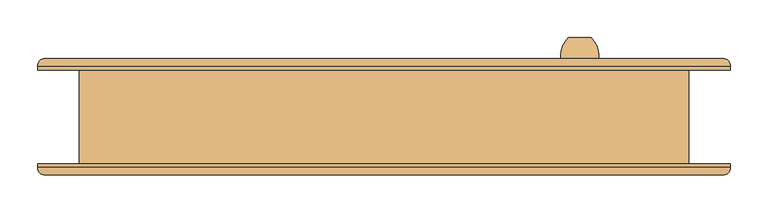
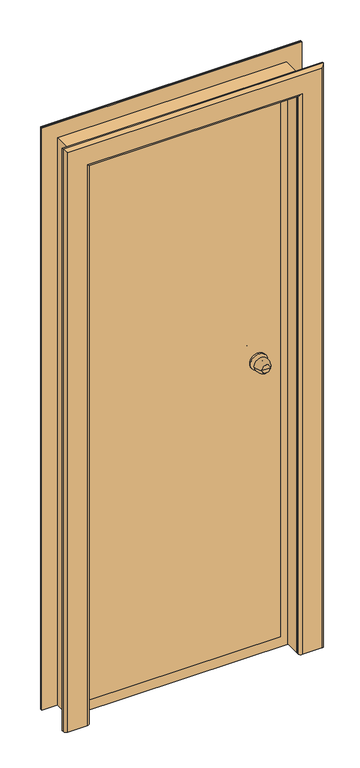
"""IFC4 building model written with IfcOpenShell, lengths in millimetres: door geometry, Наружная дверь 1-Навесная - Один проем наружу с порогом - 31173-2003 : ДСН КЛН  М1 УЗ 2100-810 ГОСТ 31173-2003."""

from ifc_helpers import new_model, si_unit, point, frame, origin, place, context, project, spatial, polyline, circle_curve, ellipse_curve, trimmed, outline, extrude, faceted_brep, source, transform, mapped, element, save
from ifc_brep_helpers import plane_surface, cylinder_surface, revolved_surface, advanced_brep


def door_b60437f9(model_context):
    return source(origin(), model_context, "Body", "SolidModel", [
        advanced_brep(
        [(245.0, 105.5, 1100.0), (275.0, 105.5, 1100.0), (260.0, 105.5, 1100.0), (235.0, 75.5, 1100.0), (285.0, 75.5, 1100.0), (242.0, 75.5, 1100.0), (278.0, 75.5, 1100.0), (250.0, 67.5, 1100.0), (270.0, 67.5, 1100.0), (250.0, 61.5, 1100.0), (270.0, 61.5, 1100.0), (290.0, 61.5, 1100.0), (230.0, 61.5, 1100.0), (290.0, 55.5, 1100.0), (230.0, 55.5, 1100.0)],
        [
            (0, 1, circle_curve(frame((260.0, 105.5, 1100.0), z_axis=(0.0, 1.0, 0.0), x_axis=(1.0, 0.0, 0.0)), 15.0)),
            (1, 2),
            (2, 0),
            (1, 0, circle_curve(frame((260.0, 105.5, 1100.0), z_axis=(0.0, 1.0, 0.0), x_axis=(1.0, 0.0, 0.0)), 15.0)),
            (0, 3, circle_curve(frame((269.6226265, 80.6257912, 1100.0), z_axis=(0.0, 0.0, 1.0), x_axis=(1.0, 0.0, 0.0)), 35.0)),
            (3, 4, circle_curve(frame((260.0, 75.5, 1100.0), z_axis=(0.0, 1.0, 0.0), x_axis=(1.0, 0.0, 0.0)), 25.0)),
            (4, 1, circle_curve(frame((250.3773735, 80.6257912, 1100.0), z_axis=(0.0, 0.0, 1.0), x_axis=(-1.0, 0.0, 0.0)), 35.0)),
            (4, 3, circle_curve(frame((260.0, 75.5, 1100.0), z_axis=(0.0, 1.0, 0.0), x_axis=(1.0, 0.0, 0.0)), 25.0)),
            (3, 5),
            (5, 6, circle_curve(frame((260.0, 75.5, 1100.0), z_axis=(0.0, 1.0, 0.0), x_axis=(1.0, 0.0, 0.0)), 18.0)),
            (6, 4),
            (6, 5, circle_curve(frame((260.0, 75.5, 1100.0), z_axis=(0.0, 1.0, 0.0), x_axis=(1.0, 0.0, 0.0)), 18.0)),
            (5, 7, circle_curve(frame((242.0, 67.5, 1100.0), z_axis=(0.0, 0.0, -1.0), x_axis=(1.0, 0.0, 0.0)), 8.0)),
            (7, 8, circle_curve(frame((260.0, 67.5, 1100.0), z_axis=(0.0, 1.0, 0.0), x_axis=(1.0, 0.0, 0.0)), 10.0)),
            (8, 6, circle_curve(frame((278.0, 67.5, 1100.0), z_axis=(0.0, 0.0, -1.0), x_axis=(-1.0, 0.0, 0.0)), 8.0)),
            (8, 7, circle_curve(frame((260.0, 67.5, 1100.0), z_axis=(0.0, 1.0, 0.0), x_axis=(1.0, 0.0, 0.0)), 10.0)),
            (7, 9),
            (9, 10, circle_curve(frame((260.0, 61.5, 1100.0), z_axis=(0.0, 1.0, 0.0), x_axis=(1.0, 0.0, 0.0)), 10.0)),
            (10, 8),
            (10, 9, circle_curve(frame((260.0, 61.5, 1100.0), z_axis=(0.0, 1.0, 0.0), x_axis=(1.0, 0.0, 0.0)), 10.0)),
            (11, 12, circle_curve(frame((260.0, 61.5, 1100.0), z_axis=(0.0, 1.0, 0.0), x_axis=(-1.0, 0.0, 0.0)), 30.0)),
            (12, 11, circle_curve(frame((260.0, 61.5, 1100.0), z_axis=(0.0, 1.0, 0.0), x_axis=(-1.0, 0.0, 0.0)), 30.0)),
            (13, 14, circle_curve(frame((260.0, 55.5, 1100.0), z_axis=(0.0, -1.0, 0.0), x_axis=(-1.0, 0.0, 0.0)), 30.0)),
            (14, 13, circle_curve(frame((260.0, 55.5, 1100.0), z_axis=(0.0, -1.0, 0.0), x_axis=(-1.0, 0.0, 0.0)), 30.0)),
            (11, 13),
            (14, 12),
        ],
        [
            plane_surface(frame((260.0, 105.5, 1100.0), z_axis=(0.0, 1.0, 0.0), x_axis=(1.0, 0.0, 0.0))),
            revolved_surface(trimmed(ellipse_curve(frame((250.3773735, 80.6257912, 1100.0), z_axis=(0.0, 0.0, -1.0), x_axis=(-1.0, 0.0, 0.0)), 35.0, 35.0), [point((275.0, 105.5, 1100.0))], [point((285.0, 75.5, 1100.0))], True, "CARTESIAN"), (260.0, 135.5, 1100.0), (0.0, -1.0, 0.0)),
            plane_surface(frame((260.0, 75.5, 1100.0), z_axis=(0.0, -1.0, 0.0), x_axis=(1.0, 0.0, 0.0))),
            revolved_surface(trimmed(ellipse_curve(frame((278.0, 67.5, 1100.0), z_axis=(0.0, 0.0, 1.0), x_axis=(-1.0, 0.0, 0.0)), 8.0, 8.0), [point((278.0, 75.5, 1100.0))], [point((270.0, 67.5, 1100.0))], True, "CARTESIAN"), (260.0, 135.5, 1100.0), (0.0, -1.0, 0.0)),
            cylinder_surface(frame((260.0, 135.5, 1100.0), z_axis=(0.0, -1.0, 0.0), x_axis=(1.0, 0.0, 0.0)), 10.0),
            plane_surface(frame((230.0, 61.5, 1100.0), z_axis=(0.0, 1.0, 0.0), x_axis=(0.0, 0.0, 1.0))),
            plane_surface(frame((230.0, 55.5, 1100.0), z_axis=(0.0, -1.0, 0.0), x_axis=(0.0, 0.0, -1.0))),
            cylinder_surface(frame((260.0, 55.5, 1100.0), z_axis=(0.0, 1.0, 0.0), x_axis=(-1.0, 0.0, 0.0)), 30.0),
        ],
        [
            (0, [[1, 2, 3]]),
            (0, [[-2, 4, -3]]),
            (1, [[-1, 5, 6, 7]]),
            (1, [[-4, -7, 8, -5]]),
            (2, [[-6, 9, 10, 11]]),
            (2, [[-8, -11, 12, -9]]),
            (3, [[-10, 13, 14, 15]]),
            (3, [[-12, -15, 16, -13]]),
            (4, [[-14, 17, 18, 19]]),
            (4, [[-16, -19, 20, -17]]),
            (5, [[21, 22], [-18, -20]]),
            (6, [[23, 24]]),
            (7, [[-21, 25, -24, 26]]),
            (7, [[-22, -26, -23, -25]]),
        ],
    ),
        advanced_brep(
        [(275.0, -64.5, 1100.0), (245.0, -64.5, 1100.0), (260.0, -64.5, 1100.0), (285.0, -34.5, 1100.0), (235.0, -34.5, 1100.0), (278.0, -34.5, 1100.0), (242.0, -34.5, 1100.0), (270.0, -26.5, 1100.0), (250.0, -26.5, 1100.0), (270.0, -20.5, 1100.0), (250.0, -20.5, 1100.0), (230.0, -20.5, 1100.0), (290.0, -20.5, 1100.0), (230.0, -14.5, 1100.0), (290.0, -14.5, 1100.0)],
        [
            (0, 1, circle_curve(frame((260.0, -64.5, 1100.0), z_axis=(0.0, -1.0, 0.0), x_axis=(-1.0, 0.0, 0.0)), 15.0)),
            (1, 2),
            (2, 0),
            (1, 0, circle_curve(frame((260.0, -64.5, 1100.0), z_axis=(0.0, -1.0, 0.0), x_axis=(-1.0, 0.0, 0.0)), 15.0)),
            (0, 3, circle_curve(frame((250.3773735, -39.6257912, 1100.0), z_axis=(0.0, 0.0, 1.0), x_axis=(-1.0, 0.0, 0.0)), 35.0)),
            (3, 4, circle_curve(frame((260.0, -34.5, 1100.0), z_axis=(0.0, -1.0, 0.0), x_axis=(-1.0, 0.0, 0.0)), 25.0)),
            (4, 1, circle_curve(frame((269.6226265, -39.6257912, 1100.0), z_axis=(0.0, 0.0, 1.0), x_axis=(1.0, 0.0, 0.0)), 35.0)),
            (4, 3, circle_curve(frame((260.0, -34.5, 1100.0), z_axis=(0.0, -1.0, 0.0), x_axis=(-1.0, 0.0, 0.0)), 25.0)),
            (3, 5),
            (5, 6, circle_curve(frame((260.0, -34.5, 1100.0), z_axis=(0.0, -1.0, 0.0), x_axis=(-1.0, 0.0, 0.0)), 18.0)),
            (6, 4),
            (6, 5, circle_curve(frame((260.0, -34.5, 1100.0), z_axis=(0.0, -1.0, 0.0), x_axis=(-1.0, 0.0, 0.0)), 18.0)),
            (5, 7, circle_curve(frame((278.0, -26.5, 1100.0), z_axis=(0.0, 0.0, -1.0), x_axis=(-1.0, 0.0, 0.0)), 8.0)),
            (7, 8, circle_curve(frame((260.0, -26.5, 1100.0), z_axis=(0.0, -1.0, 0.0), x_axis=(-1.0, 0.0, 0.0)), 10.0)),
            (8, 6, circle_curve(frame((242.0, -26.5, 1100.0), z_axis=(0.0, 0.0, -1.0), x_axis=(1.0, 0.0, 0.0)), 8.0)),
            (8, 7, circle_curve(frame((260.0, -26.5, 1100.0), z_axis=(0.0, -1.0, 0.0), x_axis=(-1.0, 0.0, 0.0)), 10.0)),
            (7, 9),
            (9, 10, circle_curve(frame((260.0, -20.5, 1100.0), z_axis=(0.0, -1.0, 0.0), x_axis=(-1.0, 0.0, 0.0)), 10.0)),
            (10, 8),
            (10, 9, circle_curve(frame((260.0, -20.5, 1100.0), z_axis=(0.0, -1.0, 0.0), x_axis=(-1.0, 0.0, 0.0)), 10.0)),
            (11, 12, circle_curve(frame((260.0, -20.5, 1100.0), z_axis=(0.0, -1.0, 0.0), x_axis=(1.0, 0.0, 0.0)), 30.0)),
            (12, 11, circle_curve(frame((260.0, -20.5, 1100.0), z_axis=(0.0, -1.0, 0.0), x_axis=(1.0, 0.0, 0.0)), 30.0)),
            (13, 14, circle_curve(frame((260.0, -14.5, 1100.0), z_axis=(0.0, 1.0, 0.0), x_axis=(1.0, 0.0, 0.0)), 30.0)),
            (14, 13, circle_curve(frame((260.0, -14.5, 1100.0), z_axis=(0.0, 1.0, 0.0), x_axis=(1.0, 0.0, 0.0)), 30.0)),
            (11, 13),
            (14, 12),
        ],
        [
            plane_surface(frame((260.0, -64.5, 1100.0), z_axis=(0.0, -1.0, 0.0), x_axis=(-1.0, 0.0, 0.0))),
            revolved_surface(trimmed(ellipse_curve(frame((269.6226265, -39.6257912, 1100.0), z_axis=(0.0, 0.0, -1.0), x_axis=(1.0, 0.0, 0.0)), 35.0, 35.0), [point((245.0, -64.5, 1100.0))], [point((235.0, -34.5, 1100.0))], True, "CARTESIAN"), (260.0, -94.5, 1100.0), (0.0, 1.0, 0.0)),
            plane_surface(frame((260.0, -34.5, 1100.0), z_axis=(0.0, 1.0, 0.0), x_axis=(-1.0, 0.0, 0.0))),
            revolved_surface(trimmed(ellipse_curve(frame((242.0, -26.5, 1100.0), z_axis=(0.0, 0.0, 1.0), x_axis=(1.0, 0.0, 0.0)), 8.0, 8.0), [point((242.0, -34.5, 1100.0))], [point((250.0, -26.5, 1100.0))], True, "CARTESIAN"), (260.0, -94.5, 1100.0), (0.0, 1.0, 0.0)),
            cylinder_surface(frame((260.0, -94.5, 1100.0), z_axis=(0.0, 1.0, 0.0), x_axis=(-1.0, 0.0, 0.0)), 10.0),
            plane_surface(frame((290.0, -20.5, 1100.0), z_axis=(0.0, -1.0, 0.0), x_axis=(0.0, 0.0, 1.0))),
            plane_surface(frame((290.0, -14.5, 1100.0), z_axis=(0.0, 1.0, 0.0), x_axis=(0.0, 0.0, -1.0))),
            cylinder_surface(frame((260.0, -14.5, 1100.0), z_axis=(0.0, -1.0, 0.0), x_axis=(1.0, 0.0, 0.0)), 30.0),
        ],
        [
            (0, [[1, 2, 3]]),
            (0, [[-2, 4, -3]]),
            (1, [[-1, 5, 6, 7]]),
            (1, [[-4, -7, 8, -5]]),
            (2, [[-6, 9, 10, 11]]),
            (2, [[-8, -11, 12, -9]]),
            (3, [[-10, 13, 14, 15]]),
            (3, [[-12, -15, 16, -13]]),
            (4, [[-14, 17, 18, 19]]),
            (4, [[-16, -19, 20, -17]]),
            (5, [[21, 22], [-18, -20]]),
            (6, [[23, 24]]),
            (7, [[-21, 25, -24, 26]]),
            (7, [[-22, -26, -23, -25]]),
        ],
    ),
        faceted_brep([(340.0, -14.5, 42.0), (-340.0, -14.5, 42.0), (-340.0, -9.5, 42.0), (340.0, -9.5, 42.0), (340.0, -14.5, 2055.0), (340.0, -9.5, 2055.0), (-340.0, -9.5, 2055.0), (320.0, -9.5, 2035.0), (-320.0, -9.5, 2035.0), (-320.0, -9.5, 62.0), (320.0, -9.5, 62.0), (-340.0, -14.5, 2055.0), (320.0, 55.5, 62.0), (320.0, 55.5, 2035.0), (-320.0, 55.5, 62.0), (-320.0, 55.5, 2035.0)], [[[0, 1, 2, 3]], [[4, 0, 3, 5]], [[5, 3, 2, 6], [7, 8, 9, 10]], [[2, 1, 11, 6]], [[11, 1, 0, 4]], [[7, 10, 12, 13]], [[9, 14, 12, 10]], [[15, 14, 9, 8]], [[13, 12, 14, 15]], [[4, 5, 6, 11]], [[7, 13, 15, 8]]]),
        extrude(outline(polyline([(0.0, 385.0), (2100.0, 385.0), (2100.0, -385.0), (0.0, -385.0), (0.0, -370.0), (2085.0, -370.0), (2085.0, 370.0), (0.0, 370.0), (0.0, 385.0)])), frame((0.0, -62.5, 0.0), z_axis=(0.0, 1.0, 0.0), x_axis=(0.0, 0.0, 1.0)), (0.0, 0.0, 1.0), 55.0),
        faceted_brep([(385.0, -7.5, 0.0), (-385.0, -7.5, 0.0), (-385.0, 62.5, 0.0), (385.0, 62.5, 0.0), (-385.0, -7.5, 2100.0), (-385.0, 62.5, 2100.0), (385.0, 62.5, 2100.0), (-305.0, 62.5, 2020.0), (-305.0, 62.5, 80.0), (305.0, 62.5, 80.0), (305.0, 62.5, 2020.0), (385.0, -7.5, 2100.0), (-325.0, -7.5, 60.0), (-325.0, -7.5, 2040.0), (325.0, -7.5, 2040.0), (325.0, -7.5, 60.0), (325.0, 57.5, 60.0), (-325.0, 57.5, 60.0), (-325.0, 57.5, 2040.0), (325.0, 57.5, 2040.0), (-305.0, 57.5, 80.0), (-305.0, 57.5, 2020.0), (305.0, 57.5, 2020.0), (305.0, 57.5, 80.0)], [[[0, 1, 2, 3]], [[1, 4, 5, 2]], [[2, 5, 6, 3], [7, 8, 9, 10]], [[4, 1, 0, 11], [12, 13, 14, 15]], [[16, 17, 12, 15]], [[17, 18, 13, 12]], [[18, 17, 16, 19], [20, 21, 22, 23]], [[9, 8, 20, 23]], [[8, 7, 21, 20]], [[11, 0, 3, 6]], [[19, 16, 15, 14]], [[10, 9, 23, 22]], [[4, 11, 6, 5]], [[18, 19, 14, 13]], [[7, 10, 22, 21]]]),
        advanced_brep(
        [(-460.0, 62.5, 0.0), (-460.0, 67.5, 0.0), (-450.0, 77.5, 0.0), (-380.0, 77.5, 0.0), (-370.0, 67.5, 0.0), (-370.0, 62.5, 0.0), (-370.0, 62.5, 2085.0), (370.0, 62.5, 2085.0), (370.0, 62.5, 0.0), (460.0, 62.5, 0.0), (460.0, 62.5, 2175.0), (-460.0, 62.5, 2175.0), (-370.0, 67.5, 2085.0), (-380.0, 77.5, 2095.0), (-450.0, 77.5, 2165.0), (450.0, 77.5, 2165.0), (450.0, 77.5, 0.0), (380.0, 77.5, 0.0), (380.0, 77.5, 2095.0), (-460.0, 67.5, 2175.0), (460.0, 67.5, 0.0), (460.0, 67.5, 2175.0), (370.0, 67.5, 0.0), (370.0, 67.5, 2085.0)],
        [
            (0, 1),
            (1, 2, circle_curve(frame((-450.0, 67.5, 0.0), z_axis=(0.0, 0.0, -1.0), x_axis=(-1.0, 0.0, 0.0)), 10.0)),
            (2, 3),
            (3, 4, circle_curve(frame((-380.0, 67.5, 0.0), z_axis=(0.0, 0.0, -1.0), x_axis=(-1.0, 0.0, 0.0)), 10.0)),
            (4, 5),
            (5, 0),
            (5, 6),
            (6, 7),
            (7, 8),
            (8, 9),
            (9, 10),
            (10, 11),
            (11, 0),
            (4, 12),
            (12, 6),
            (3, 13),
            (13, 12, ellipse_curve(frame((-380.0, 67.5, 2095.0), z_axis=(-0.7071067811865475, 0.0, -0.7071067811865475), x_axis=(0.7071067811865474, 0.0, -0.7071067811865476)), 14.1421356, 10.0)),
            (2, 14),
            (14, 15),
            (15, 16),
            (16, 17),
            (17, 18),
            (18, 13),
            (1, 19),
            (19, 14, ellipse_curve(frame((-450.0, 67.5, 2165.0), z_axis=(-0.7071067811865475, 0.0, -0.7071067811865475), x_axis=(0.7071067811865474, 0.0, -0.7071067811865476)), 14.1421356, 10.0)),
            (11, 19),
            (9, 20),
            (20, 21),
            (21, 10),
            (8, 22),
            (22, 17, circle_curve(frame((380.0, 67.5, 0.0), z_axis=(0.0, 0.0, -1.0), x_axis=(1.0, 0.0, 0.0)), 10.0)),
            (16, 20, circle_curve(frame((450.0, 67.5, 0.0), z_axis=(0.0, 0.0, -1.0), x_axis=(1.0, 0.0, 0.0)), 10.0)),
            (23, 22),
            (7, 23),
            (23, 18, ellipse_curve(frame((380.0, 67.5, 2095.0), z_axis=(0.7071067811865475, 0.0, -0.7071067811865475), x_axis=(0.7071067811865474, 0.0, 0.7071067811865476)), 14.1421356, 10.0)),
            (15, 21, ellipse_curve(frame((450.0, 67.5, 2165.0), z_axis=(0.7071067811865475, 0.0, -0.7071067811865475), x_axis=(0.7071067811865474, 0.0, 0.7071067811865476)), 14.1421356, 10.0)),
            (12, 23),
            (19, 21),
        ],
        [
            plane_surface(frame((-405.0, 62.5, 0.0), z_axis=(0.0, 0.0, -1.0), x_axis=(0.0, 1.0, 0.0))),
            plane_surface(frame((-460.0, 62.5, 0.0), z_axis=(0.0, -1.0, 0.0), x_axis=(0.0, 0.0, 1.0))),
            plane_surface(frame((-370.0, 62.5, 0.0), z_axis=(1.0, 0.0, 0.0), x_axis=(0.0, 0.0, 1.0))),
            cylinder_surface(frame((-380.0, 67.5, 0.0), z_axis=(0.0, 0.0, -1.0), x_axis=(-1.0, 0.0, 0.0)), 10.0),
            plane_surface(frame((-380.0, 77.5, 0.0), z_axis=(0.0, 1.0, 0.0), x_axis=(0.0, 0.0, 1.0))),
            cylinder_surface(frame((-450.0, 67.5, 0.0), z_axis=(0.0, 0.0, -1.0), x_axis=(-1.0, 0.0, 0.0)), 10.0),
            plane_surface(frame((-460.0, 67.5, 0.0), z_axis=(-1.0, 0.0, 0.0), x_axis=(0.0, 0.0, 1.0))),
            plane_surface(frame((460.0, 67.5, 2175.0), z_axis=(1.0, 0.0, 0.0), x_axis=(0.0, 0.0, -1.0))),
            plane_surface(frame((405.0, 62.5, 0.0), z_axis=(0.0, 0.0, -1.0), x_axis=(0.0, 1.0, 0.0))),
            plane_surface(frame((370.0, 62.5, 2085.0), z_axis=(-1.0, 0.0, 0.0), x_axis=(0.0, 0.0, -1.0))),
            cylinder_surface(frame((380.0, 67.5, 2120.0), z_axis=(0.0, 0.0, 1.0), x_axis=(1.0, 0.0, 0.0)), 10.0),
            cylinder_surface(frame((450.0, 67.5, 2120.0), z_axis=(0.0, 0.0, 1.0), x_axis=(1.0, 0.0, 0.0)), 10.0),
            plane_surface(frame((-370.0, 62.5, 2085.0), z_axis=(0.0, 0.0, -1.0), x_axis=(1.0, 0.0, 0.0))),
            cylinder_surface(frame((-405.0, 67.5, 2095.0), z_axis=(-1.0, 0.0, 0.0), x_axis=(0.0, 0.0, 1.0)), 10.0),
            cylinder_surface(frame((-405.0, 67.5, 2165.0), z_axis=(-1.0, 0.0, 0.0), x_axis=(0.0, 0.0, 1.0)), 10.0),
            plane_surface(frame((-460.0, 67.5, 2175.0), z_axis=(0.0, 0.0, 1.0), x_axis=(1.0, 0.0, 0.0))),
        ],
        [
            (0, [[1, 2, 3, 4, 5, 6]]),
            (1, [[7, 8, 9, 10, 11, 12, 13, -6]]),
            (2, [[14, 15, -7, -5]]),
            (3, [[16, 17, -14, -4]]),
            (4, [[18, 19, 20, 21, 22, 23, -16, -3]]),
            (5, [[24, 25, -18, -2]]),
            (6, [[-13, 26, -24, -1]]),
            (7, [[-11, 27, 28, 29]]),
            (8, [[-10, 30, 31, -21, 32, -27]]),
            (9, [[33, -30, -9, 34]]),
            (10, [[-22, -31, -33, 35]]),
            (11, [[-28, -32, -20, 36]]),
            (12, [[37, -34, -8, -15]]),
            (13, [[-23, -35, -37, -17]]),
            (14, [[38, -36, -19, -25]]),
            (15, [[-12, -29, -38, -26]]),
        ],
    ),
        advanced_brep(
        [(460.0, -62.5, 0.0), (460.0, -67.5, 0.0), (450.0, -77.5, 0.0), (380.0, -77.5, 0.0), (370.0, -67.5, 0.0), (370.0, -62.5, 0.0), (370.0, -62.5, 2085.0), (-370.0, -62.5, 2085.0), (-370.0, -62.5, 0.0), (-460.0, -62.5, 0.0), (-460.0, -62.5, 2175.0), (460.0, -62.5, 2175.0), (370.0, -67.5, 2085.0), (380.0, -77.5, 2095.0), (450.0, -77.5, 2165.0), (-450.0, -77.5, 2165.0), (-450.0, -77.5, 0.0), (-380.0, -77.5, 0.0), (-380.0, -77.5, 2095.0), (460.0, -67.5, 2175.0), (-460.0, -67.5, 0.0), (-460.0, -67.5, 2175.0), (-370.0, -67.5, 0.0), (-370.0, -67.5, 2085.0)],
        [
            (0, 1),
            (1, 2, circle_curve(frame((450.0, -67.5, 0.0), z_axis=(0.0, 0.0, -1.0), x_axis=(1.0, 0.0, 0.0)), 10.0)),
            (2, 3),
            (3, 4, circle_curve(frame((380.0, -67.5, 0.0), z_axis=(0.0, 0.0, -1.0), x_axis=(1.0, 0.0, 0.0)), 10.0)),
            (4, 5),
            (5, 0),
            (5, 6),
            (6, 7),
            (7, 8),
            (8, 9),
            (9, 10),
            (10, 11),
            (11, 0),
            (4, 12),
            (12, 6),
            (3, 13),
            (13, 12, ellipse_curve(frame((380.0, -67.5, 2095.0), z_axis=(0.7071067811865475, 0.0, -0.7071067811865475), x_axis=(-0.7071067811865474, 0.0, -0.7071067811865476)), 14.1421356, 10.0)),
            (2, 14),
            (14, 15),
            (15, 16),
            (16, 17),
            (17, 18),
            (18, 13),
            (1, 19),
            (19, 14, ellipse_curve(frame((450.0, -67.5, 2165.0), z_axis=(0.7071067811865475, 0.0, -0.7071067811865475), x_axis=(-0.7071067811865474, 0.0, -0.7071067811865476)), 14.1421356, 10.0)),
            (11, 19),
            (9, 20),
            (20, 21),
            (21, 10),
            (8, 22),
            (22, 17, circle_curve(frame((-380.0, -67.5, 0.0), z_axis=(0.0, 0.0, -1.0), x_axis=(-1.0, 0.0, 0.0)), 10.0)),
            (16, 20, circle_curve(frame((-450.0, -67.5, 0.0), z_axis=(0.0, 0.0, -1.0), x_axis=(-1.0, 0.0, 0.0)), 10.0)),
            (23, 22),
            (7, 23),
            (23, 18, ellipse_curve(frame((-380.0, -67.5, 2095.0), z_axis=(-0.7071067811865475, 0.0, -0.7071067811865475), x_axis=(-0.7071067811865474, 0.0, 0.7071067811865476)), 14.1421356, 10.0)),
            (15, 21, ellipse_curve(frame((-450.0, -67.5, 2165.0), z_axis=(-0.7071067811865475, 0.0, -0.7071067811865475), x_axis=(-0.7071067811865474, 0.0, 0.7071067811865476)), 14.1421356, 10.0)),
            (12, 23),
            (19, 21),
        ],
        [
            plane_surface(frame((405.0, -62.5, 0.0), z_axis=(0.0, 0.0, -1.0), x_axis=(0.0, 1.0, 0.0))),
            plane_surface(frame((460.0, -62.5, 0.0), z_axis=(0.0, 1.0, 0.0), x_axis=(0.0, 0.0, 1.0))),
            plane_surface(frame((370.0, -62.5, 0.0), z_axis=(-1.0, 0.0, 0.0), x_axis=(0.0, 0.0, 1.0))),
            cylinder_surface(frame((380.0, -67.5, 0.0), z_axis=(0.0, 0.0, -1.0), x_axis=(1.0, 0.0, 0.0)), 10.0),
            plane_surface(frame((380.0, -77.5, 0.0), z_axis=(0.0, -1.0, 0.0), x_axis=(0.0, 0.0, 1.0))),
            cylinder_surface(frame((450.0, -67.5, 0.0), z_axis=(0.0, 0.0, -1.0), x_axis=(1.0, 0.0, 0.0)), 10.0),
            plane_surface(frame((460.0, -67.5, 0.0), z_axis=(1.0, 0.0, 0.0), x_axis=(0.0, 0.0, 1.0))),
            plane_surface(frame((-460.0, -67.5, 2175.0), z_axis=(-1.0, 0.0, 0.0), x_axis=(0.0, 0.0, -1.0))),
            plane_surface(frame((-405.0, -62.5, 0.0), z_axis=(0.0, 0.0, -1.0), x_axis=(0.0, 1.0, 0.0))),
            plane_surface(frame((-370.0, -62.5, 2085.0), z_axis=(1.0, 0.0, 0.0), x_axis=(0.0, 0.0, -1.0))),
            cylinder_surface(frame((-380.0, -67.5, 2120.0), z_axis=(0.0, 0.0, 1.0), x_axis=(-1.0, 0.0, 0.0)), 10.0),
            cylinder_surface(frame((-450.0, -67.5, 2120.0), z_axis=(0.0, 0.0, 1.0), x_axis=(-1.0, 0.0, 0.0)), 10.0),
            plane_surface(frame((370.0, -62.5, 2085.0), z_axis=(0.0, 0.0, -1.0), x_axis=(-1.0, 0.0, 0.0))),
            cylinder_surface(frame((405.0, -67.5, 2095.0), z_axis=(1.0, 0.0, 0.0), x_axis=(0.0, 0.0, 1.0)), 10.0),
            cylinder_surface(frame((405.0, -67.5, 2165.0), z_axis=(1.0, 0.0, 0.0), x_axis=(0.0, 0.0, 1.0)), 10.0),
            plane_surface(frame((460.0, -67.5, 2175.0), z_axis=(0.0, 0.0, 1.0), x_axis=(-1.0, 0.0, 0.0))),
        ],
        [
            (0, [[1, 2, 3, 4, 5, 6]]),
            (1, [[7, 8, 9, 10, 11, 12, 13, -6]]),
            (2, [[14, 15, -7, -5]]),
            (3, [[16, 17, -14, -4]]),
            (4, [[18, 19, 20, 21, 22, 23, -16, -3]]),
            (5, [[24, 25, -18, -2]]),
            (6, [[-13, 26, -24, -1]]),
            (7, [[-11, 27, 28, 29]]),
            (8, [[-10, 30, 31, -21, 32, -27]]),
            (9, [[33, -30, -9, 34]]),
            (10, [[-22, -31, -33, 35]]),
            (11, [[-28, -32, -20, 36]]),
            (12, [[37, -34, -8, -15]]),
            (13, [[-23, -35, -37, -17]]),
            (14, [[38, -36, -19, -25]]),
            (15, [[-12, -29, -38, -26]]),
        ],
    ),
        extrude(outline(polyline([(0.0, 405.0), (2120.0, 405.0), (2120.0, -405.0), (0.0, -405.0), (0.0, -385.0), (2100.0, -385.0), (2100.0, 385.0), (0.0, 385.0), (0.0, 405.0)])), frame((0.0, -62.5, 0.0), z_axis=(0.0, 1.0, 0.0), x_axis=(0.0, 0.0, 1.0)), (0.0, 0.0, 1.0), 125.0),
    ])


if __name__ == "__main__":
    model = new_model("IFC4")
    model_context = context("Model", 3, world=origin())
    ifc_project = project(units=[si_unit("LENGTHUNIT", "METRE", prefix="MILLI")], contexts=[model_context])
    site = spatial("IfcSite", under=ifc_project)
    building = spatial("IfcBuilding", under=site)
    placement = place(None, origin())
    door_shape = door_b60437f9(model_context)
    element("IfcDoor", 1, ObjectType="Наружная дверь 1-Навесная - Один проем наружу с порогом - 31173-2003 : ДСН КЛН  М1 УЗ 2100-810 ГОСТ 31173-2003", at=placement, inside=building, context=model_context, shape_type="MappedRepresentation", body=[
        mapped(door_shape, transform((0.0, 0.0, 0.0), x_axis=(1.0, 0.0, 0.0), y_axis=(0.0, 1.0, 0.0), z_axis=(0.0, 0.0, 1.0))),
    ])
    save(model, "model.ifc")

# Revit data of these elements
# Type "Наружная дверь 1-Навесная - Один проем наружу с порогом - 31173-2003 : ДСН КЛН  М1 УЗ 2100-810 ГОСТ 31173-2003"
#   Type Mark = "153"
#   Description = "ДСН КЛН  М1 УЗ 2100-900 ГОСТ 31173-2003"
#   Проекционное соединение по ширине = 90 mm
#   Rough Width = 810 mm
#   Rough Height = 2120 mm
#   Угол проема [instance default] = 30°
#   Толщина_Тепл_Изоляции = 20 mm
#   Heat Transfer Coefficient (U) = 3.7021 W/(m²·K)
#   Height = 2100 mm
#   Width = 770 mm
#   Ширина каркаса = 60 mm
#   Толщина каркаса = 70 mm
#   Вставка двери [instance default] = 0 mm
#   Правая сторона = no
#   Левая сторона = yes
#   Function = 1
#   Обрезка = Сталь
#   Панель = Сталь
#   Тепловая изоляция = Тепловая изоляция
#   Кадр = Сталь
#   Дверная ручка = Металл
#   Visual Light Transmittance = 0
#   Solar Heat Gain Coefficient = 0
#   Construction Type Id = ""
#   Wall Closure = (empty or 0)
#   Analytic Construction = (empty or 0)
# Element 1 (IfcDoor, "Наружная дверь 1-Навесная - Один проем наружу с порогом - 31173-2003 : ДСН КЛН  М1 УЗ 2100-810 ГОСТ 31173-2003")
#   Materials on its faces: "Сталь", "Металл", "Тепловая изоляция"
# Materials
#   "Сталь": class "Металл", colour RGB 247 247 247, transparency 0
#   "Тепловая изоляция": class "Пластмасса", colour RGB 185 154 119, transparency 0, Cost = 0
#   "Металл": class "Металл", colour RGB 249 249 249, transparency 0
